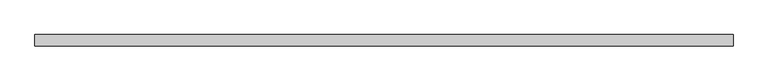
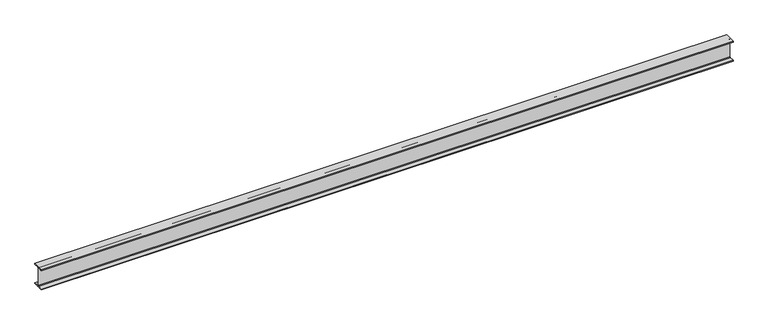
"""IFC4 building model written with IfcOpenShell, lengths in millimetres: beam geometry, Old_Steel Beam_H-KSD3502 : H_SB_ASB_H-488×300x11x18."""

from ifc_helpers import new_model, si_unit, point, frame, frame_2d, origin, place, context, project, spatial, polyline, circle_curve, trimmed, segment, composite_curve, outline, extrude, source, transform, mapped, element, save


def beam_41ab70f5(model_context):
    return source(origin(), model_context, "Body", "SweptSolid", [
        extrude(outline(composite_curve([segment(polyline([(82.5, -141.5), (82.5, -151.7), (-82.5, -151.7), (-82.5, -141.5), (-11.9, -141.5)]), True, "CONTINUOUS"), segment(trimmed(circle_curve(frame_2d((-11.9, -132.6)), 8.9), [point((-11.9, -141.5))], [point((-3.0, -132.6))], True, "CARTESIAN"), True, "CONTINUOUS"), segment(polyline([(-3.0, -132.6), (-3.0, 132.6)]), True, "CONTINUOUS"), segment(trimmed(circle_curve(frame_2d((-11.9, 132.6)), 8.9), [point((-3.0, 132.6))], [point((-11.9, 141.5))], True, "CARTESIAN"), True, "CONTINUOUS"), segment(polyline([(-11.9, 141.5), (-82.5, 141.5), (-82.5, 151.7), (82.5, 151.7), (82.5, 141.5), (11.9, 141.5)]), True, "CONTINUOUS"), segment(trimmed(circle_curve(frame_2d((11.9, 132.6)), 8.9), [point((11.9, 141.5))], [point((3.0, 132.6))], True, "CARTESIAN"), True, "CONTINUOUS"), segment(polyline([(3.0, 132.6), (3.0, -132.6)]), True, "CONTINUOUS"), segment(trimmed(circle_curve(frame_2d((11.9, -132.6)), 8.9), [point((3.0, -132.6))], [point((11.9, -141.5))], True, "CARTESIAN"), True, "CONTINUOUS"), segment(polyline([(11.9, -141.5), (82.5, -141.5)]), True, "CONTINUOUS")], self_intersect=False)), frame((-5029.8, 0.0, 0.0), z_axis=(1.0, 0.0, 0.0), x_axis=(0.0, 1.0, 0.0)), (0.0, 0.0, 1.0), 10059.6),
    ])


if __name__ == "__main__":
    model = new_model("IFC4")
    model_context = context("Model", 3, world=origin())
    ifc_project = project(units=[si_unit("LENGTHUNIT", "METRE", prefix="MILLI")], contexts=[model_context])
    site = spatial("IfcSite", under=ifc_project)
    building = spatial("IfcBuilding", under=site)
    placement = place(None, origin())
    beam_shape = beam_41ab70f5(model_context)
    element("IfcBeam", 1, ObjectType="Old_Steel Beam_H-KSD3502 : H_SB_ASB_H-488×300x11x18", at=placement, inside=building, context=model_context, shape_type="MappedRepresentation", body=[
        mapped(beam_shape, transform((0.0, 0.0, 0.0), x_axis=(1.0, 0.0, 0.0), y_axis=(0.0, 1.0, 0.0), z_axis=(0.0, 0.0, 1.0))),
    ])
    save(model, "model.ifc")

# Revit data of these elements
# Type "Old_Steel Beam_H-KSD3502 : H_SB_ASB_H-488×300x11x18"
#   Width = 30.0 cm
#   Web Thickness = 1.1 cm
#   Web Fillet = 2.6 cm
#   Warping Constant = 4473230.0 cm⁶
#   Torsional Moment of Inertia = 137.492 cm⁴
#   Torsional Modulus = 1.0 cm³
#   Section Area = 163.5 cm²
#   Plastic Modulus weak axis = 830.0 cm³
#   Plastic Modulus strong axis = 3230.0 cm³
#   Perimeter = 2.11 m²/m
#   Nominal Weight = 128.00 kgf/m
#   Moment of Inertia weak axis = 8110.00 cm⁴
#   Moment of Inertia strong axis = 71000.00 cm⁴
#   Height = 48.8 cm
#   Flange Thickness = 1.8 cm
#   Elastic Modulus weak axis = 541.0 cm³
#   Elastic Modulus strong axis = 2910.0 cm³
#   Centroid Vertical = 24.4 cm
#   Centroid Horizontal = 15.0 cm
#   Length [instance default] = 1.5240 m
#   Structural Material [instance default] = Steel, 45-345
#   Assembly Code = ""
# Element 1 (IfcBeam, "Old_Steel Beam_H-KSD3502 : H_SB_ASB_H-488×300x11x18")
#   Structural Material = none
# Materials
#   "Steel, 45-345": class "Metal", colour RGB 189 187 185, transparency 0, Description = "Steel 345 MPa", Cost = 0
